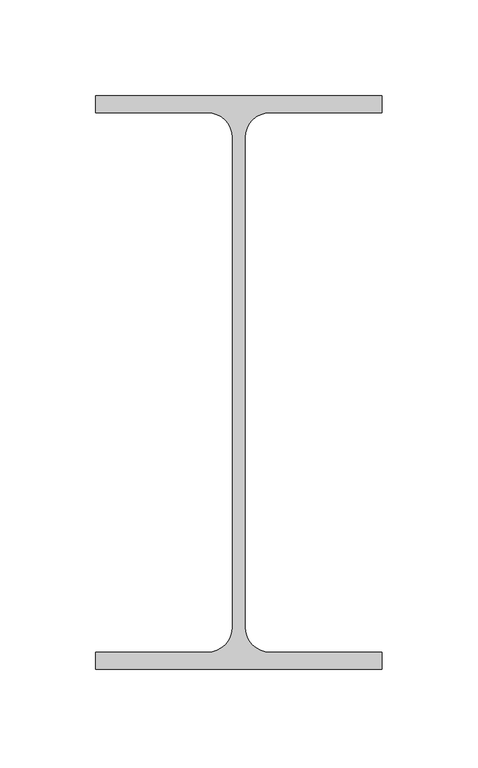
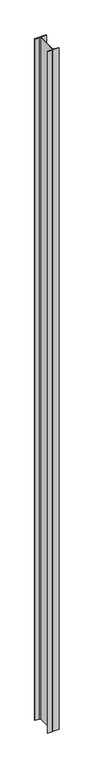
"""IFC4 building model written with IfcOpenShell, lengths in millimetres: column geometry, Steel Column_H_KS : H_SC_AR_S01_H-300x150x6.5x9_SSC1."""

from ifc_helpers import new_model, si_unit, point, frame, frame_2d, origin, place, context, project, spatial, polyline, circle_curve, trimmed, segment, composite_curve, outline, extrude, source, transform, mapped, element, save


def column_fef3e922(model_context):
    return source(origin(), model_context, "Body", "SweptSolid", [
        extrude(outline(composite_curve([segment(polyline([(75.0, 150.0), (75.0, 141.0), (16.25, 141.0)]), True, "CONTINUOUS"), segment(trimmed(circle_curve(frame_2d((16.25, 128.0)), 13.0), [point((16.25, 141.0))], [point((3.25, 128.0))], True, "CARTESIAN"), True, "CONTINUOUS"), segment(polyline([(3.25, 128.0), (3.25, -128.0)]), True, "CONTINUOUS"), segment(trimmed(circle_curve(frame_2d((16.25, -128.0)), 13.0), [point((3.25, -128.0))], [point((16.25, -141.0))], True, "CARTESIAN"), True, "CONTINUOUS"), segment(polyline([(16.25, -141.0), (75.0, -141.0), (75.0, -150.0), (-75.0, -150.0), (-75.0, -141.0), (-16.25, -141.0)]), True, "CONTINUOUS"), segment(trimmed(circle_curve(frame_2d((-16.25, -128.0)), 13.0), [point((-16.25, -141.0))], [point((-3.25, -128.0))], True, "CARTESIAN"), True, "CONTINUOUS"), segment(polyline([(-3.25, -128.0), (-3.25, 128.0)]), True, "CONTINUOUS"), segment(trimmed(circle_curve(frame_2d((-16.25, 128.0)), 13.0), [point((-3.25, 128.0))], [point((-16.25, 141.0))], True, "CARTESIAN"), True, "CONTINUOUS"), segment(polyline([(-16.25, 141.0), (-75.0, 141.0), (-75.0, 150.0), (75.0, 150.0)]), True, "CONTINUOUS")], self_intersect=False)), frame((0.0, 0.0, 249.9618634), z_axis=(0.0, 0.0, 1.0), x_axis=(1.0, 0.0, 0.0)), (0.0, 0.0, 1.0), 9550.0),
    ])


if __name__ == "__main__":
    model = new_model("IFC4")
    model_context = context("Model", 3, world=origin())
    ifc_project = project(units=[si_unit("LENGTHUNIT", "METRE", prefix="MILLI")], contexts=[model_context])
    site = spatial("IfcSite", under=ifc_project)
    building = spatial("IfcBuilding", under=site)
    placement = place(None, origin())
    column_shape = column_fef3e922(model_context)
    element("IfcColumn", 1, ObjectType="Steel Column_H_KS : H_SC_AR_S01_H-300x150x6.5x9_SSC1", at=placement, inside=building, context=model_context, shape_type="MappedRepresentation", body=[
        mapped(column_shape, transform((0.0, 0.0, 0.0), x_axis=(1.0, 0.0, 0.0), y_axis=(0.0, 1.0, 0.0), z_axis=(0.0, 0.0, 1.0))),
    ])
    save(model, "model.ifc")

# Revit data of these elements
# Type "Steel Column_H_KS : H_SC_AR_S01_H-300x150x6.5x9_SSC1"
#   Type Comments = "MAIN"
#   Type Mark = "SSC1"
#   H_SectionID = "H-300x150x6.5x9"
#   H_Ratio for Additional Steel Plate = 0.2
#   Width = 15.0 cm
#   Web Thickness = 0.65 cm
#   Web Fillet = 1.3 cm
#   Warping Constant = 107174.4 cm⁶
#   Torsional Moment of Inertia = 9.95386 cm⁴
#   Section Area = 46.78 cm²
#   Plastic Modulus weak axis = 105.0 cm³
#   Plastic Modulus strong axis = 542.0 cm³
#   Perimeter = 1.165 m²/m
#   Nominal Weight = 36.70 kgf/m
#   Moment of Inertia weak axis = 508.00 cm⁴
#   Moment of Inertia strong axis = 7210.00 cm⁴
#   Height = 30.0 cm
#   Flange Thickness = 0.9 cm
#   Elastic Modulus weak axis = 67.7 cm³
#   Elastic Modulus strong axis = 481.0 cm³
#   Centroid Vertical = 15.0 cm
#   Centroid Horizontal = 7.5 cm
#   Structural Material [instance default] = Steel, 45-345
#   Section Name Key = ""
#   Bolt Spacing = 0
#   Assembly Code = ""
# Element 1 (IfcColumn, "Steel Column_H_KS : H_SC_AR_S01_H-300x150x6.5x9_SSC1")
#   Materials on its faces: "Steel, 45-345"
# Materials
#   "Steel, 45-345": class "Metal", colour RGB 189 187 185, transparency 0, Description = "Steel 345 MPa", Cost = 0
